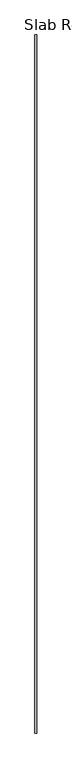
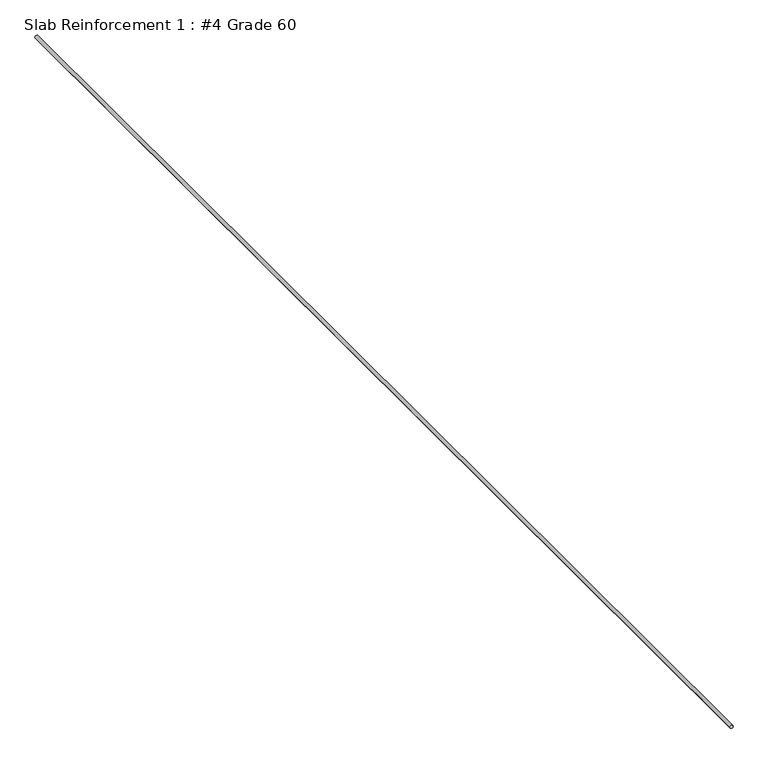
"""IFC4 building model written with IfcOpenShell, lengths in millimetres: proxy geometry, Slab Reinforcement 1 : #4 Grade 60."""

from ifc_helpers import new_model, si_unit, point, frame, frame_2d, origin, place, context, project, spatial, circle_curve, trimmed, segment, composite_curve, outline, extrude, source, transform, mapped, element, save


def slab_reinforcement_1_4_grade_60_b1e4fe1f(model_context):
    return source(origin(), model_context, "Body", "SweptSolid", [
        extrude(outline(composite_curve([segment(trimmed(circle_curve(frame_2d((-69.85, 588840.1672365)), 6.35), [point((-69.85, 588833.8172365))], [point((-69.85, 588846.5172365))], False, "CARTESIAN"), True, "CONTINUOUS"), segment(trimmed(circle_curve(frame_2d((-69.85, 588840.1672365)), 6.35), [point((-69.85, 588846.5172365))], [point((-69.85, 588833.8172365))], False, "CARTESIAN"), True, "CONTINUOUS")], self_intersect=False)), frame((0.0, -536411.2413841, 0.0), z_axis=(0.0, 1.0, 0.0), x_axis=(0.0, 0.0, 1.0)), (0.0, 0.0, 1.0), 4724.4),
    ])


if __name__ == "__main__":
    model = new_model("IFC4")
    model_context = context("Model", 3, world=origin())
    ifc_project = project(units=[si_unit("LENGTHUNIT", "METRE", prefix="MILLI")], contexts=[model_context])
    site = spatial("IfcSite", under=ifc_project)
    building = spatial("IfcBuilding", under=site)
    placement = place(None, origin())
    slab_reinforcement_1_4_grade_60_shape = slab_reinforcement_1_4_grade_60_b1e4fe1f(model_context)
    element("IfcBuildingElementProxy", 1, Name="Slab Reinforcement 1 : #4 Grade 60", ObjectType="Slab Reinforcement 1 : #4 Grade 60", at=placement, inside=building, context=model_context, shape_type="MappedRepresentation", body=[
        mapped(slab_reinforcement_1_4_grade_60_shape, transform((0.0, 0.0, 0.0), x_axis=(1.0, 0.0, 0.0), y_axis=(0.0, 1.0, 0.0), z_axis=(0.0, 0.0, 1.0))),
    ])
    save(model, "model.ifc")

# Revit data of these elements
# Element 1 (IfcBuildingElementProxy, "Slab Reinforcement 1 : #4 Grade 60")
#   Materials on its faces: "#4 GR. 60 REINF. @ 16\" O.C. EW."
# Materials
#   "#4 GR. 60 REINF. @ 16\" O.C. EW.": class "Generic", colour RGB 84 83 81, transparency 0, Cost = 0
